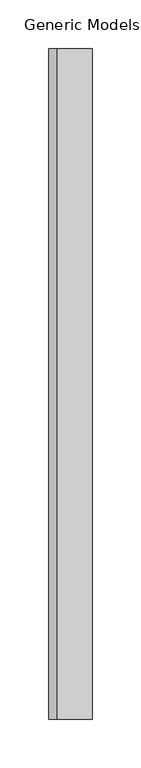
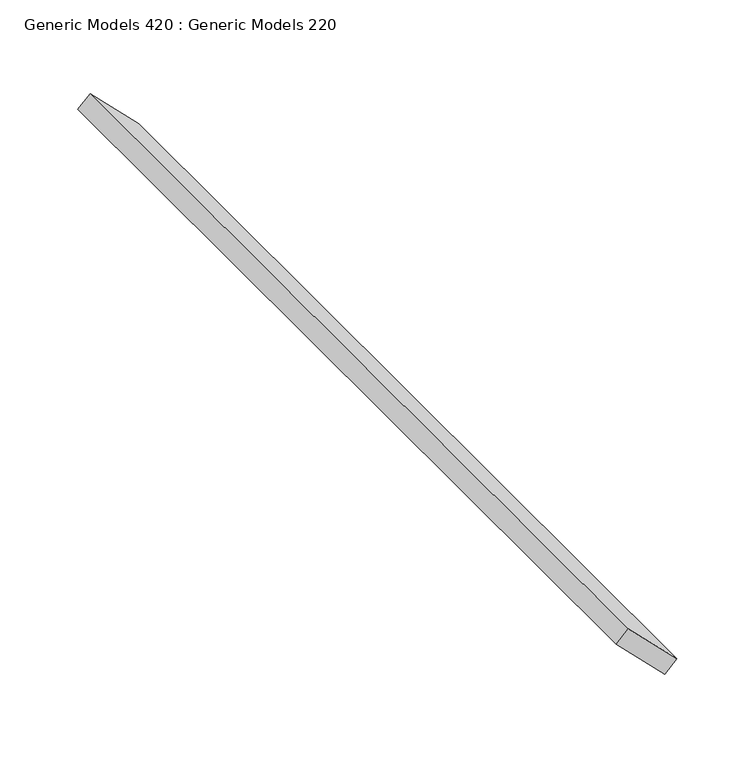
"""IFC4 building model written with IfcOpenShell, lengths in millimetres: proxy geometry, Generic Models 420 : Generic Models 220."""

from ifc_helpers import new_model, si_unit, frame, origin, place, context, project, spatial, polyline, outline, extrude, source, transform, mapped, element, save


def generic_models_420_generic_models_220_60c5558d(model_context):
    return source(origin(), model_context, "Body", "SweptSolid", [
        extrude(outline(polyline([(0.0, -50.8), (0.0, 0.0), (690.8142348, 0.0), (690.8142348, -50.8), (0.0, -50.8)])), frame((-6899.085451, -4564.8872686, 128640.6762561), z_axis=(0.7071067811865582, 0.0, 0.7071067811865369), x_axis=(0.0, 1.0, 0.0)), (0.0, 0.0, 1.0), 12.7),
    ])


if __name__ == "__main__":
    model = new_model("IFC4")
    model_context = context("Model", 3, world=origin())
    ifc_project = project(units=[si_unit("LENGTHUNIT", "METRE", prefix="MILLI")], contexts=[model_context])
    site = spatial("IfcSite", under=ifc_project)
    building = spatial("IfcBuilding", under=site)
    placement = place(None, origin())
    generic_models_420_generic_models_220_shape = generic_models_420_generic_models_220_60c5558d(model_context)
    element("IfcBuildingElementProxy", 1, Name="Generic Models 420 : Generic Models 220", ObjectType="Generic Models 420 : Generic Models 220", at=placement, inside=building, context=model_context, shape_type="MappedRepresentation", body=[
        mapped(generic_models_420_generic_models_220_shape, transform((0.0, 0.0, 0.0), x_axis=(1.0, 0.0, 0.0), y_axis=(0.0, 1.0, 0.0), z_axis=(0.0, 0.0, 1.0))),
    ])
    save(model, "model.ifc")

# Revit data of these elements
# Element 1 (IfcBuildingElementProxy, "Generic Models 420 : Generic Models 220")
#   Materials on its faces: "_WOOD TONE ALUMINUM EXTRUSION SLAT BY KNOTWOOD"
# Materials
#   "_WOOD TONE ALUMINUM EXTRUSION SLAT BY KNOTWOOD": class "Generic", colour RGB 177 130 114, transparency 0, Cost = 0
